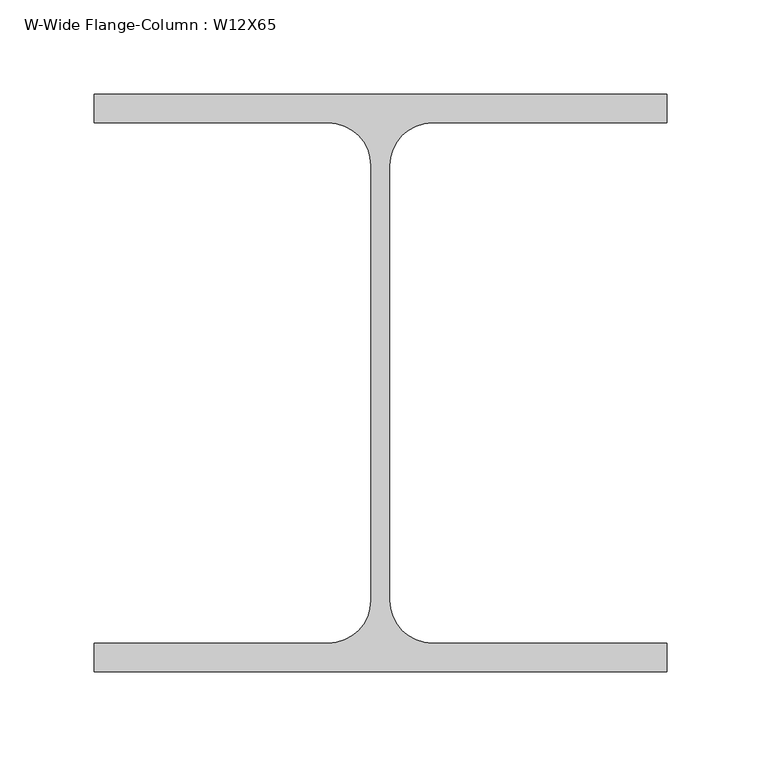
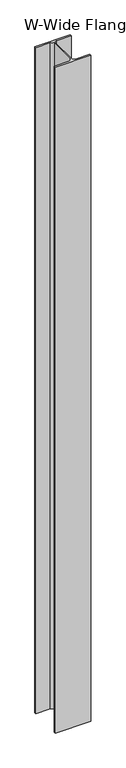
"""IFC4 building model written with IfcOpenShell, lengths in millimetres: column geometry, W-Wide Flange-Column : W12X65."""

from ifc_helpers import new_model, si_unit, point, frame, frame_2d, origin, place, context, project, spatial, polyline, circle_curve, trimmed, segment, composite_curve, outline, extrude, source, transform, mapped, element, save


def w_wide_flange_column_w12x65_ce0bf66e(model_context):
    return source(origin(), model_context, "Body", "SweptSolid", [
        extrude(outline(composite_curve([segment(polyline([(152.4, 153.67), (152.4, 138.303), (27.686, 138.303)]), True, "CONTINUOUS"), segment(trimmed(circle_curve(frame_2d((27.686, 115.57)), 22.733), [point((27.686, 138.303))], [point((4.953, 115.57))], True, "CARTESIAN"), True, "CONTINUOUS"), segment(polyline([(4.953, 115.57), (4.953, -115.57)]), True, "CONTINUOUS"), segment(trimmed(circle_curve(frame_2d((27.686, -115.57)), 22.733), [point((4.953, -115.57))], [point((27.686, -138.303))], True, "CARTESIAN"), True, "CONTINUOUS"), segment(polyline([(27.686, -138.303), (152.4, -138.303), (152.4, -153.67), (-152.4, -153.67), (-152.4, -138.303), (-27.686, -138.303)]), True, "CONTINUOUS"), segment(trimmed(circle_curve(frame_2d((-27.686, -115.57)), 22.733), [point((-27.686, -138.303))], [point((-4.953, -115.57))], True, "CARTESIAN"), True, "CONTINUOUS"), segment(polyline([(-4.953, -115.57), (-4.953, 115.57)]), True, "CONTINUOUS"), segment(trimmed(circle_curve(frame_2d((-27.686, 115.57)), 22.733), [point((-4.953, 115.57))], [point((-27.686, 138.303))], True, "CARTESIAN"), True, "CONTINUOUS"), segment(polyline([(-27.686, 138.303), (-152.4, 138.303), (-152.4, 153.67), (152.4, 153.67)]), True, "CONTINUOUS")], self_intersect=False)), frame((0.0, 0.0, 11550.65), z_axis=(0.0, 0.0, 1.0), x_axis=(1.0, 0.0, 0.0)), (0.0, 0.0, 1.0), 6076.95),
    ])


if __name__ == "__main__":
    model = new_model("IFC4")
    model_context = context("Model", 3, world=origin())
    ifc_project = project(units=[si_unit("LENGTHUNIT", "METRE", prefix="MILLI")], contexts=[model_context])
    site = spatial("IfcSite", under=ifc_project)
    building = spatial("IfcBuilding", under=site)
    placement = place(None, origin())
    w_wide_flange_column_w12x65_shape = w_wide_flange_column_w12x65_ce0bf66e(model_context)
    element("IfcColumn", 1, ObjectType="W-Wide Flange-Column : W12X65", at=placement, inside=building, context=model_context, shape_type="MappedRepresentation", body=[
        mapped(w_wide_flange_column_w12x65_shape, transform((0.0, 0.0, 0.0), x_axis=(1.0, 0.0, 0.0), y_axis=(0.0, 1.0, 0.0), z_axis=(0.0, 0.0, 1.0))),
    ])
    save(model, "model.ifc")

# Revit data of these elements
# Type "W-Wide Flange-Column : W12X65"
#   Assembly Code = "B10"
#   W = 65
#   bf = 1' - 0"
#   d = 1' - 0.1"
#   k = 0' - 1 1/2"
#   kr = 0' - 0.895"
#   tf = 0' - 0.605"
#   tw = 0' - 0.39"
#   A = 0.132639 SF
#   Structural Material [instance default] = Steel ASTM A992
# Element 1 (IfcColumn, "W-Wide Flange-Column : W12X65")
#   Materials on its faces: "Steel ASTM A992"
# Materials
#   "Steel ASTM A992": class "Metal", colour RGB 199 199 199, transparency 0, Description = "Structural steel 50ksi", Cost = 0
